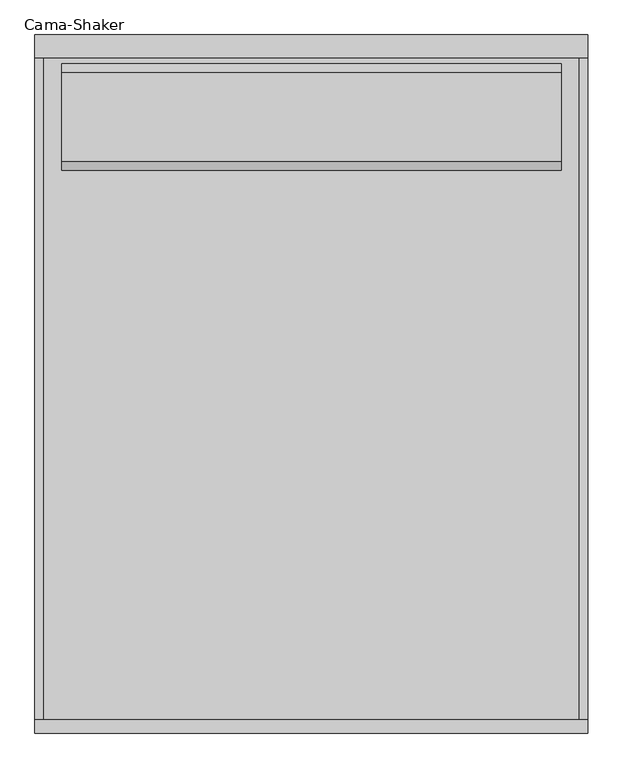
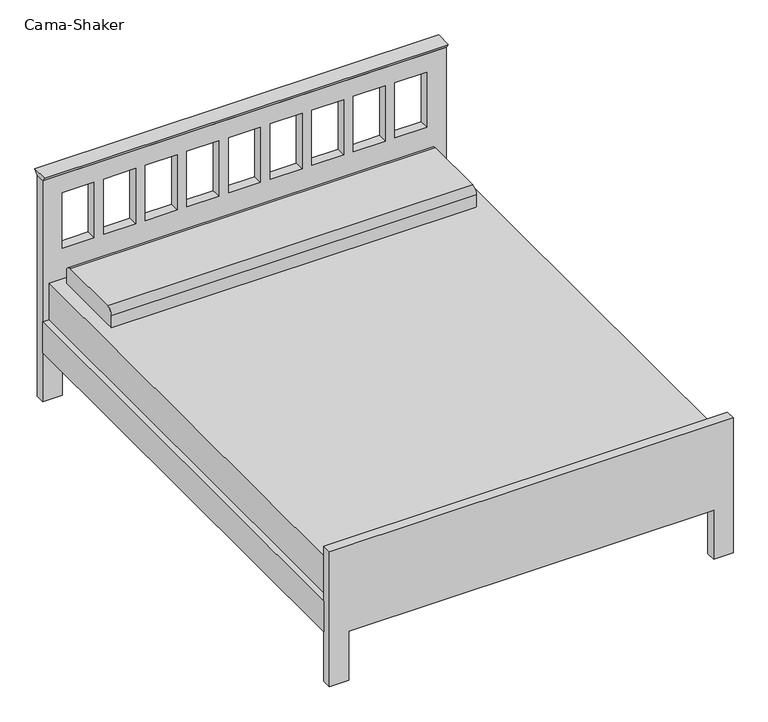
"""IFC4 building model written with IfcOpenShell, lengths in millimetres: furniture geometry, Cama-Shaker : 1580 x 1981 mm - Casal 3."""

from ifc_helpers import new_model, si_unit, point, frame, frame_2d, origin, place, context, project, spatial, polyline, circle_curve, trimmed, segment, composite_curve, outline, extrude, source, transform, mapped, element, save


def cama_shaker_1ce55566(model_context):
    return source(origin(), model_context, "Body", "SweptSolid", [
        extrude(outline(polyline([(-38.1, 914.4), (-51.9545455, 933.45), (13.8545455, 933.45), (0.0, 914.4), (-38.1, 914.4)])), frame((-808.8365546, 0.0, 0.0), z_axis=(1.0, 0.0, 0.0), x_axis=(0.0, 1.0, 0.0)), (0.0, 0.0, 1.0), 1580.0533613),
        extrude(outline(composite_curve([segment(polyline([(-373.2486637, 482.6), (-373.2486637, 533.4)]), True, "CONTINUOUS"), segment(trimmed(circle_curve(frame_2d((-347.8486637, 533.4)), 25.4), [point((-373.2486637, 533.4))], [point((-347.8486637, 558.8))], False, "CARTESIAN"), True, "CONTINUOUS"), segment(polyline([(-347.8486637, 558.8), (-93.8486637, 558.8)]), True, "CONTINUOUS"), segment(trimmed(circle_curve(frame_2d((-93.8486637, 533.4)), 25.4), [point((-93.8486637, 558.8))], [point((-68.4486637, 533.4))], False, "CARTESIAN"), True, "CONTINUOUS"), segment(polyline([(-68.4486637, 533.4), (-68.4486637, 482.6), (-373.2486637, 482.6)]), True, "CONTINUOUS")], self_intersect=False)), frame((-732.85, 0.0, 0.0), z_axis=(1.0, 0.0, 0.0), x_axis=(0.0, 1.0, 0.0)), (0.0, 0.0, 1.0), 1427.6),
        extrude(outline(polyline([(745.55, -38.1), (745.55, -1943.1), (-783.65, -1943.1), (-783.65, -38.1), (745.55, -38.1)])), frame((0.0, 0.0, 228.6), z_axis=(0.0, 0.0, 1.0), x_axis=(1.0, 0.0, 0.0)), (0.0, 0.0, 1.0), 254.0),
        extrude(outline(polyline([(745.55, -1943.1), (745.55, -38.1), (770.95, -38.1), (770.95, -1943.1), (745.55, -1943.1)])), frame((0.0, 0.0, 203.0994861), z_axis=(0.0, 0.0, 1.0), x_axis=(1.0, 0.0, 0.0)), (0.0, 0.0, 1.0), 127.0),
        extrude(outline(polyline([(-809.05, -1943.1), (-809.05, -38.1), (-783.65, -38.1), (-783.65, -1943.1), (-809.05, -1943.1)])), frame((0.0, 0.0, 203.5755296), z_axis=(0.0, 0.0, 1.0), x_axis=(1.0, 0.0, 0.0)), (0.0, 0.0, 1.0), 127.0),
        extrude(outline(polyline([(0.0, -732.85), (203.2, -732.85), (203.2, 694.75), (0.0, 694.75), (0.0, 770.95), (558.8, 770.95), (558.8, -809.05), (0.0, -809.05), (0.0, -732.85)])), frame((0.0, -1981.2, 0.0), z_axis=(0.0, 1.0, 0.0), x_axis=(0.0, 0.0, 1.0)), (0.0, 0.0, 1.0), 38.1),
        extrude(outline(polyline([(914.4, 771.2168067), (914.4, -808.8365546), (0.0, -808.8365546), (0.0, -732.85), (203.2, -732.85), (203.2, 694.75), (0.0, 694.75), (0.0, 771.2168067), (914.4, 771.2168067)]), holes=[polyline([(838.2, -608.0944444), (609.6, -608.0944444), (609.6, -732.85), (838.2, -732.85), (838.2, -608.0944444)]), polyline([(838.2, -445.2388889), (609.6, -445.2388889), (609.6, -569.9944444), (838.2, -569.9944444), (838.2, -445.2388889)]), polyline([(838.2, -282.3833333), (609.6, -282.3833333), (609.6, -407.1388889), (838.2, -407.1388889), (838.2, -282.3833333)]), polyline([(838.2, -119.5277778), (609.6, -119.5277778), (609.6, -244.2833333), (838.2, -244.2833333), (838.2, -119.5277778)]), polyline([(838.2, 206.1833333), (609.6, 206.1833333), (609.6, 81.4277778), (838.2, 81.4277778), (838.2, 206.1833333)]), polyline([(838.2, 369.0388889), (609.6, 369.0388889), (609.6, 244.2833333), (838.2, 244.2833333), (838.2, 369.0388889)]), polyline([(838.2, 531.8944444), (609.6, 531.8944444), (609.6, 407.1388889), (838.2, 407.1388889), (838.2, 531.8944444)]), polyline([(838.2, 694.75), (609.6, 694.75), (609.6, 569.9944444), (838.2, 569.9944444), (838.2, 694.75)]), polyline([(838.2, 43.3277778), (609.6, 43.3277778), (609.6, -81.4277778), (838.2, -81.4277778), (838.2, 43.3277778)])]), frame((0.0, -38.1, 0.0), z_axis=(0.0, 1.0, 0.0), x_axis=(0.0, 0.0, 1.0)), (0.0, 0.0, 1.0), 38.1),
    ])


if __name__ == "__main__":
    model = new_model("IFC4")
    model_context = context("Model", 3, world=origin())
    ifc_project = project(units=[si_unit("LENGTHUNIT", "METRE", prefix="MILLI")], contexts=[model_context])
    site = spatial("IfcSite", under=ifc_project)
    building = spatial("IfcBuilding", under=site)
    placement = place(None, origin())
    cama_shaker_shape = cama_shaker_1ce55566(model_context)
    element("IfcFurniture", 1, ObjectType="Cama-Shaker : 1580 x 1981 mm - Casal 3", at=placement, inside=building, context=model_context, shape_type="MappedRepresentation", body=[
        mapped(cama_shaker_shape, transform((0.0, 0.0, 0.0), x_axis=(1.0, 0.0, 0.0), y_axis=(0.0, 1.0, 0.0), z_axis=(0.0, 0.0, 1.0))),
    ])
    save(model, "model.ifc")

# Revit data of these elements
# Project information
#   Data de emissão do projeto = "Data de emissão"
#   Status do projeto = "Status do projeto"
#   Nome do cliente = "Proprietário"
#   Endereço do projeto = "## Rua\nCidade, Estado  Cep"
#   Nome do projeto = "Nome do projeto"
#   Número do projeto = "0001"
# Type "Cama-Shaker : 1580 x 1981 mm - Casal 3"
#   Comprimento = 1.9812 m
#   Largura = 1.58 m
#   Material da moldura = wood brown
#   Material do colchão = Linho, branco
#   Default Elevation = 0
# Element 1 (IfcFurniture, "Cama-Shaker : 1580 x 1981 mm - Casal 3")
#   Materials on its faces: "wood brown", "Linho, branco"
# Materials
#   "wood brown": class "Wood", colour RGB 80 39 12, transparency 0, Cost = 0
#   "Linho, branco": class "Tecido", colour RGB 247 247 239, transparency 0, Description = "Linho, branco", Cost = 0
